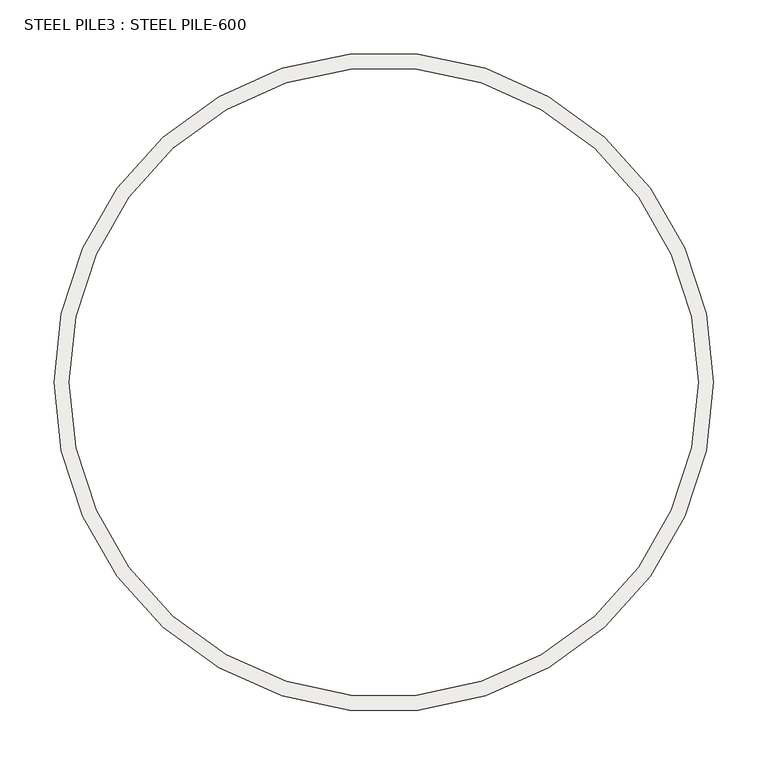
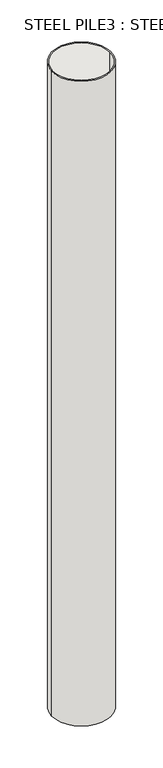
"""IFC4 building model written with IfcOpenShell, lengths in millimetres: slab geometry, STEEL PILE3 : STEEL PILE-600."""

from ifc_helpers import new_model, si_unit, point, frame, frame_2d, origin, place, context, project, spatial, circle_curve, trimmed, segment, composite_curve, outline, extrude, source, transform, mapped, element, save


def steel_pile3_steel_pile_600_5de2f451(model_context):
    return source(origin(), model_context, "Body", "SweptSolid", [
        extrude(outline(composite_curve([segment(trimmed(circle_curve(frame_2d((-30945.7763606, -7583.9705533)), 304.5), [point((-31250.2763606, -7583.9705533))], [point((-30641.2763606, -7583.9705533))], False, "CARTESIAN"), True, "CONTINUOUS"), segment(trimmed(circle_curve(frame_2d((-30945.7763606, -7583.9705533)), 304.5), [point((-30641.2763606, -7583.9705533))], [point((-31250.2763606, -7583.9705533))], False, "CARTESIAN"), True, "CONTINUOUS")], self_intersect=False), holes=[composite_curve([segment(trimmed(circle_curve(frame_2d((-30945.7763606, -7583.9705533)), 290.5), [point((-31236.2763606, -7583.9705533))], [point((-30655.2763606, -7583.9705533))], True, "CARTESIAN"), True, "CONTINUOUS"), segment(trimmed(circle_curve(frame_2d((-30945.7763606, -7583.9705533)), 290.5), [point((-30655.2763606, -7583.9705533))], [point((-31236.2763606, -7583.9705533))], True, "CARTESIAN"), True, "CONTINUOUS")], self_intersect=False)]), frame((0.0, 0.0, -6850.0), z_axis=(0.0, 0.0, 1.0), x_axis=(1.0, 0.0, 0.0)), (0.0, 0.0, 1.0), 7000.0),
    ])


if __name__ == "__main__":
    model = new_model("IFC4")
    model_context = context("Model", 3, world=origin())
    ifc_project = project(units=[si_unit("LENGTHUNIT", "METRE", prefix="MILLI")], contexts=[model_context])
    site = spatial("IfcSite", under=ifc_project)
    building = spatial("IfcBuilding", under=site)
    placement = place(None, origin())
    steel_pile3_steel_pile_600_shape = steel_pile3_steel_pile_600_5de2f451(model_context)
    element("IfcSlab", 1, ObjectType="STEEL PILE3 : STEEL PILE-600", at=placement, inside=building, context=model_context, shape_type="MappedRepresentation", body=[
        mapped(steel_pile3_steel_pile_600_shape, transform((0.0, 0.0, 0.0), x_axis=(1.0, 0.0, 0.0), y_axis=(0.0, 1.0, 0.0), z_axis=(0.0, 0.0, 1.0))),
    ])
    save(model, "model.ifc")
